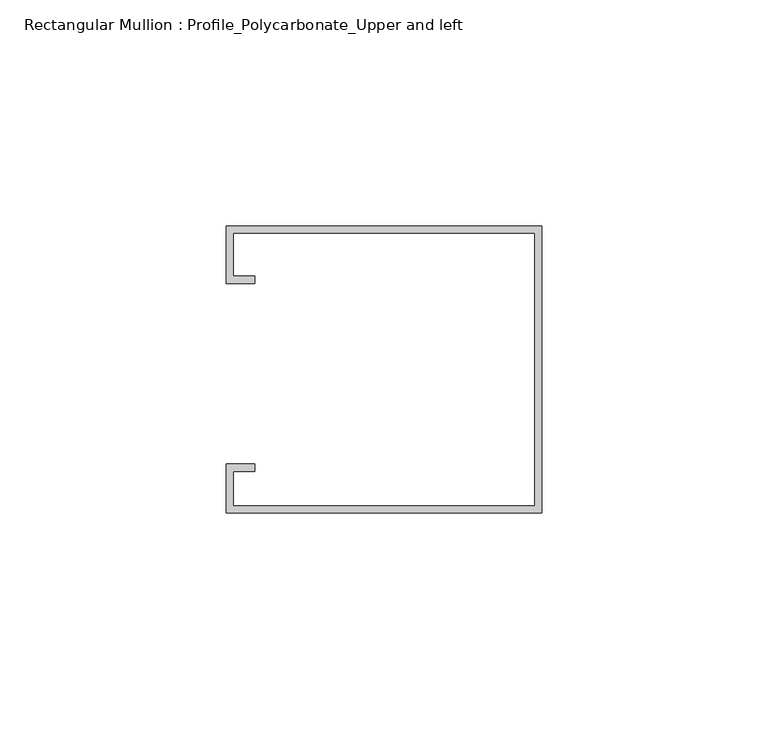
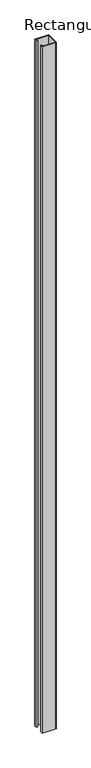
"""IFC4 building model written with IfcOpenShell, lengths in millimetres: member geometry, Rectangular Mullion : Profile_Polycarbonate_Upper and left."""

import ifcopenshell
import ifcopenshell.guid

model = None  # the IFC model being written
_history = None  # IfcOwnerHistory: only IFC2X3 demands one
_inside = {}  # id of a spatial element -> (the spatial element, [elements in it])
_under = {}  # id of a project, library or spatial element -> (it, [spatial elements below it])
_declared = {}  # id of a project -> (the project, [libraries it declares])
_typed = {}  # id of a type object -> (the type object, [elements of that type])
_made_of = {}  # id of a material, layer set ... -> (it, [elements and type objects made of it])


def new_model(schema):
    """Start an empty IFC model of exactly this schema.

    Asked for "IFC4X3", IfcOpenShell would pick the latest addendum, in which some entities
    have other attributes; the version numbers below select the first issue.
    IFC2X3 requires an IfcOwnerHistory on every rooted entity: one is made here for all.
    """
    global model, _history
    if schema == "IFC4X3":
        model = ifcopenshell.file(schema_version=(4, 3, 0, 0))
    else:
        model = ifcopenshell.file(schema=schema)
    _inside.clear()
    _under.clear()
    _declared.clear()
    _typed.clear()
    _made_of.clear()
    _history = None
    if model.schema == "IFC2X3":
        org = make("IfcOrganization", Name="unknown")
        user = make(
            "IfcPersonAndOrganization",
            ThePerson=make("IfcPerson", FamilyName="unknown"),
            TheOrganization=org,
        )
        app = make(
            "IfcApplication",
            ApplicationDeveloper=org,
            Version="unknown",
            ApplicationFullName="unknown",
            ApplicationIdentifier="unknown",
        )
        _history = make(
            "IfcOwnerHistory",
            OwningUser=user,
            OwningApplication=app,
            ChangeAction="ADDED",
            CreationDate=0,
        )
    return model


def make(cls, **values):
    """One entity of the class cls with the attributes given. An attribute that is None is left unset."""
    return model.create_entity(
        cls, **{name: value for name, value in values.items() if value is not None}
    )


def rooted(cls, **values):
    """An entity with a GlobalId (a new one), such as an element, a storey or a relation."""
    return make(cls, GlobalId=ifcopenshell.guid.new(), OwnerHistory=_history, **values)


def si_unit(unit_type, name, prefix=None):
    """IfcSIUnit, for example si_unit("LENGTHUNIT", "METRE", prefix="MILLI")."""
    return make("IfcSIUnit", UnitType=unit_type, Prefix=prefix, Name=name)


def assignment(units):
    """IfcUnitAssignment: the units of a project."""
    return None if units is None else make("IfcUnitAssignment", Units=units)


def point(xyz):
    """IfcCartesianPoint."""
    return None if xyz is None else make("IfcCartesianPoint", Coordinates=xyz)


def direction(xyz):
    """IfcDirection."""
    return None if xyz is None else make("IfcDirection", DirectionRatios=xyz)


def frame(location, z_axis=None, x_axis=None):
    """IfcAxis2Placement3D, a coordinate frame: its origin and axes. An axis left out is left unset."""
    return make(
        "IfcAxis2Placement3D",
        Location=point(location),
        Axis=direction(z_axis),
        RefDirection=direction(x_axis),
    )


def origin():
    """The frame at (0, 0, 0) with its axes left unset."""
    return frame((0.0, 0.0, 0.0))


def place(relative_to, where):
    """IfcLocalPlacement: puts the frame where relative to a parent placement (None: the world)."""
    return make(
        "IfcLocalPlacement", PlacementRelTo=relative_to, RelativePlacement=where
    )


def context(
    kind, dimensions, precision=None, world=None, true_north=None, identifier=None
):
    """IfcGeometricRepresentationContext, for example the 3D "Model" context."""
    return make(
        "IfcGeometricRepresentationContext",
        ContextIdentifier=identifier,
        ContextType=kind,
        CoordinateSpaceDimension=dimensions,
        Precision=precision,
        WorldCoordinateSystem=world,
        TrueNorth=true_north,
    )


def project(units=None, contexts=None):
    """IfcProject with its units and contexts."""
    return rooted(
        "IfcProject",
        Name="project",
        RepresentationContexts=contexts,
        UnitsInContext=assignment(units),
    )


def spatial(cls, under=None, at=None, **own):
    """A site, building, storey or space (cls), placed at a placement, below another one or the project."""
    s = rooted(cls, ObjectPlacement=at, **own)
    if under is not None:
        _under.setdefault(under.id(), (under, []))[1].append(s)
    return s


def polyline(points):
    """IfcPolyline through the points."""
    return make("IfcPolyline", Points=[point(p) for p in points])


def outline(outer, holes=None, kind="AREA"):
    """IfcArbitraryClosedProfileDef: a profile drawn as a closed curve; with holes, ...WithVoids."""
    if holes is None:
        return make("IfcArbitraryClosedProfileDef", ProfileType=kind, OuterCurve=outer)
    return make(
        "IfcArbitraryProfileDefWithVoids",
        ProfileType=kind,
        OuterCurve=outer,
        InnerCurves=holes,
    )


def extrude(swept, where, along, depth):
    """IfcExtrudedAreaSolid: the profile swept, set in the frame where, extruded along a direction by depth."""
    return make(
        "IfcExtrudedAreaSolid",
        SweptArea=swept,
        Position=where,
        ExtrudedDirection=direction(along),
        Depth=depth,
    )


def shape(context_of_items, identifier, shape_type, items):
    """IfcShapeRepresentation: the items that make up one representation, for example the "Body"."""
    return make(
        "IfcShapeRepresentation",
        ContextOfItems=context_of_items,
        RepresentationIdentifier=identifier,
        RepresentationType=shape_type,
        Items=items,
    )


def source(mapping_origin, context_of_items, identifier, shape_type, items):
    """IfcRepresentationMap: a shape defined once, which mapped items show again and again."""
    return make(
        "IfcRepresentationMap",
        MappingOrigin=mapping_origin,
        MappedRepresentation=shape(context_of_items, identifier, shape_type, items),
    )


def transform(
    local_origin,
    x_axis=None,
    y_axis=None,
    z_axis=None,
    scale=None,
    scale2=None,
    scale3=None,
    uniform=True,
):
    """IfcCartesianTransformationOperator3D, or its non-uniform kind. x_axis, y_axis, z_axis: its Axis1, 2, 3."""
    if uniform:
        return make(
            "IfcCartesianTransformationOperator3D",
            Axis1=direction(x_axis),
            Axis2=direction(y_axis),
            LocalOrigin=point(local_origin),
            Scale=scale,
            Axis3=direction(z_axis),
        )
    return make(
        "IfcCartesianTransformationOperator3DnonUniform",
        Axis1=direction(x_axis),
        Axis2=direction(y_axis),
        LocalOrigin=point(local_origin),
        Scale=scale,
        Axis3=direction(z_axis),
        Scale2=scale2,
        Scale3=scale3,
    )


def mapped(mapping_source, mapping_target):
    """IfcMappedItem: shows the shape of a source again, moved by a transform."""
    return make(
        "IfcMappedItem", MappingSource=mapping_source, MappingTarget=mapping_target
    )


def made_of(thing, what):
    """Note that an element or type object is made of a material, layer set ...; save() writes the relation."""
    if what is not None:
        _made_of.setdefault(what.id(), (what, []))[1].append(thing)
    return thing


def element(
    cls,
    number,
    at=None,
    inside=None,
    cuts=None,
    type_object=None,
    material=None,
    context=None,
    identifier="Body",
    shape_type=None,
    held_by="IfcProductDefinitionShape",
    body=None,
    shapes=None,
    **own,
):
    """One element of the class cls, such as IfcWall. Its Tag is "e" and its number.

    at: its placement. inside: the storey or other place that contains it. cuts: it is an
    opening in that element (IfcRelVoidsElement). A single representation is given by context,
    identifier, shape_type and body (its items); several are given by shapes. held_by: the class
    of the entity that holds the representations. save() writes the other relations.
    """
    e = rooted(cls, Tag="e%d" % number, ObjectPlacement=at, **own)
    if body is not None:
        shapes = [shape(context, identifier, shape_type, body)]
    if shapes is not None:
        e.Representation = make(held_by, Representations=shapes)
    if inside is not None:
        _inside.setdefault(inside.id(), (inside, []))[1].append(e)
    if cuts is not None:
        rooted(
            "IfcRelVoidsElement", RelatingBuildingElement=cuts, RelatedOpeningElement=e
        )
    if type_object is not None:
        _typed.setdefault(type_object.id(), (type_object, []))[1].append(e)
    return made_of(e, material)


def aggregate(whole, parts):
    """IfcRelAggregates: a whole, such as a stair, and the parts it consists of."""
    return rooted("IfcRelAggregates", RelatingObject=whole, RelatedObjects=parts)


def save(model, path):
    """Write the relations noted so far, then the file.

    IfcRelAggregates (storeys below a building ...), IfcRelContainedInSpatialStructure (elements
    in a storey), IfcRelDefinesByType, IfcRelAssociatesMaterial and IfcRelDeclares: one each for
    every whole, place, type object, material and project.
    """
    for whole, parts in _under.values():
        aggregate(whole, parts)
    for where, things in _inside.values():
        rooted(
            "IfcRelContainedInSpatialStructure",
            RelatedElements=things,
            RelatingStructure=where,
        )
    for kind, things in _typed.values():
        rooted("IfcRelDefinesByType", RelatedObjects=things, RelatingType=kind)
    for what, things in _made_of.values():
        rooted("IfcRelAssociatesMaterial", RelatedObjects=things, RelatingMaterial=what)
    for by, libraries in _declared.values():
        rooted("IfcRelDeclares", RelatingContext=by, RelatedDefinitions=libraries)
    model.write(path)


def rectangular_mullion_profile_polycarbonate_upper_and_left_ee42aaf8(model_context):
    return source(origin(), model_context, "Body", "SweptSolid", [
        extrude(outline(polyline([(0.0, 32.7), (0.0, -30.8), (-69.85, -30.8), (-69.85, -20.0), (-63.5, -20.0), (-63.5, -21.5875), (-68.2625, -21.5875), (-68.2625, -29.2125), (-1.5875, -29.2125), (-1.5875, 31.1125), (-68.2625, 31.1125), (-68.2625, 21.5875), (-63.5, 21.5875), (-63.5, 20.0), (-69.85, 20.0), (-69.85, 32.7), (0.0, 32.7)])), frame((0.0, 0.0, -3657.6), z_axis=(0.0, 0.0, 1.0), x_axis=(1.0, 0.0, 0.0)), (0.0, 0.0, 1.0), 3657.6),
    ])


if __name__ == "__main__":
    model = new_model("IFC4")
    model_context = context("Model", 3, world=origin())
    ifc_project = project(units=[si_unit("LENGTHUNIT", "METRE", prefix="MILLI")], contexts=[model_context])
    site = spatial("IfcSite", under=ifc_project)
    building = spatial("IfcBuilding", under=site)
    placement = place(None, origin())
    rectangular_mullion_profile_polycarbonate_upper_and_left_shape = rectangular_mullion_profile_polycarbonate_upper_and_left_ee42aaf8(model_context)
    element("IfcMember", 1, ObjectType="Rectangular Mullion : Profile_Polycarbonate_Upper and left", at=placement, inside=building, context=model_context, shape_type="MappedRepresentation", body=[
        mapped(rectangular_mullion_profile_polycarbonate_upper_and_left_shape, transform((0.0, 0.0, 0.0), x_axis=(1.0, 0.0, 0.0), y_axis=(0.0, 1.0, 0.0), z_axis=(0.0, 0.0, 1.0))),
    ])
    save(model, "model.ifc")

# Revit data of these elements
# Type "Rectangular Mullion : Profile_Polycarbonate_Upper and left"
#   built-in parameter 1007322 = 0.208333 (stored number, unit not read)
#   built-in parameter 1007321 = 0.00520833 (stored number, unit not read)
#   built-in parameter 1007320 = 0 (stored number, unit not read)
# Element 1 (IfcMember, "Rectangular Mullion : Profile_Polycarbonate_Upper and left")
#   Materials on its faces: "ALUMINUM PROFILE AT POLYCARBONATE PANEL"
# Materials
#   "ALUMINUM PROFILE AT POLYCARBONATE PANEL": class "Metal", colour RGB 244 244 244, transparency 0, Description = "Aluminum 6061", Cost = 0
